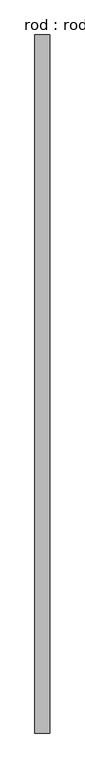
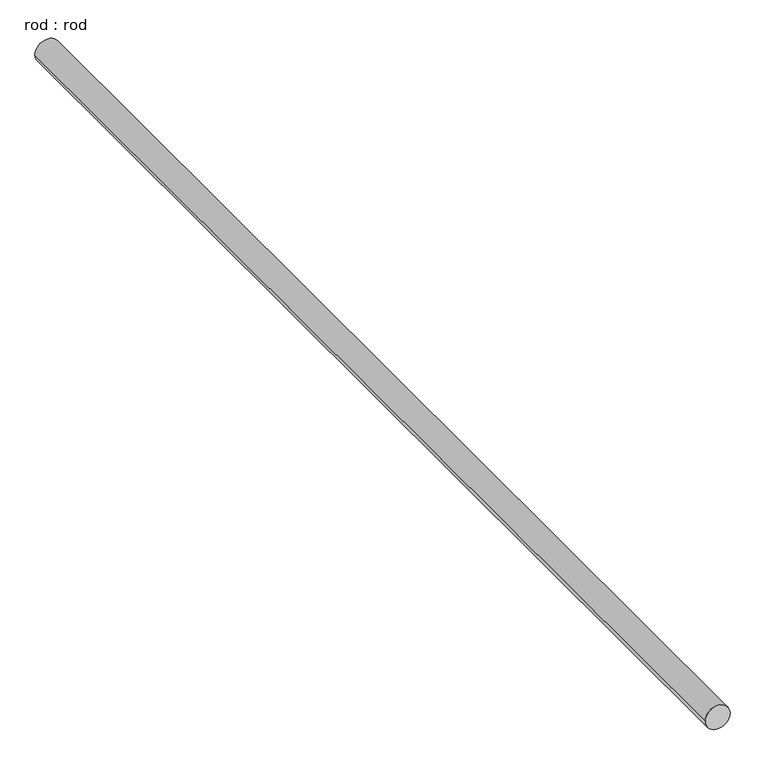
"""IFC4 building model written with IfcOpenShell, lengths in millimetres: proxy geometry, rod : rod."""

import ifcopenshell
import ifcopenshell.guid

model = None  # the IFC model being written
_history = None  # IfcOwnerHistory: only IFC2X3 demands one
_inside = {}  # id of a spatial element -> (the spatial element, [elements in it])
_under = {}  # id of a project, library or spatial element -> (it, [spatial elements below it])
_declared = {}  # id of a project -> (the project, [libraries it declares])
_typed = {}  # id of a type object -> (the type object, [elements of that type])
_made_of = {}  # id of a material, layer set ... -> (it, [elements and type objects made of it])


def new_model(schema):
    """Start an empty IFC model of exactly this schema.

    Asked for "IFC4X3", IfcOpenShell would pick the latest addendum, in which some entities
    have other attributes; the version numbers below select the first issue.
    IFC2X3 requires an IfcOwnerHistory on every rooted entity: one is made here for all.
    """
    global model, _history
    if schema == "IFC4X3":
        model = ifcopenshell.file(schema_version=(4, 3, 0, 0))
    else:
        model = ifcopenshell.file(schema=schema)
    _inside.clear()
    _under.clear()
    _declared.clear()
    _typed.clear()
    _made_of.clear()
    _history = None
    if model.schema == "IFC2X3":
        org = make("IfcOrganization", Name="unknown")
        user = make(
            "IfcPersonAndOrganization",
            ThePerson=make("IfcPerson", FamilyName="unknown"),
            TheOrganization=org,
        )
        app = make(
            "IfcApplication",
            ApplicationDeveloper=org,
            Version="unknown",
            ApplicationFullName="unknown",
            ApplicationIdentifier="unknown",
        )
        _history = make(
            "IfcOwnerHistory",
            OwningUser=user,
            OwningApplication=app,
            ChangeAction="ADDED",
            CreationDate=0,
        )
    return model


def make(cls, **values):
    """One entity of the class cls with the attributes given. An attribute that is None is left unset."""
    return model.create_entity(
        cls, **{name: value for name, value in values.items() if value is not None}
    )


def rooted(cls, **values):
    """An entity with a GlobalId (a new one), such as an element, a storey or a relation."""
    return make(cls, GlobalId=ifcopenshell.guid.new(), OwnerHistory=_history, **values)


def si_unit(unit_type, name, prefix=None):
    """IfcSIUnit, for example si_unit("LENGTHUNIT", "METRE", prefix="MILLI")."""
    return make("IfcSIUnit", UnitType=unit_type, Prefix=prefix, Name=name)


def assignment(units):
    """IfcUnitAssignment: the units of a project."""
    return None if units is None else make("IfcUnitAssignment", Units=units)


def point(xyz):
    """IfcCartesianPoint."""
    return None if xyz is None else make("IfcCartesianPoint", Coordinates=xyz)


def direction(xyz):
    """IfcDirection."""
    return None if xyz is None else make("IfcDirection", DirectionRatios=xyz)


def frame(location, z_axis=None, x_axis=None):
    """IfcAxis2Placement3D, a coordinate frame: its origin and axes. An axis left out is left unset."""
    return make(
        "IfcAxis2Placement3D",
        Location=point(location),
        Axis=direction(z_axis),
        RefDirection=direction(x_axis),
    )


def frame_2d(location, x_axis=None):
    """IfcAxis2Placement2D, a coordinate frame in the plane: its origin and x axis."""
    return make(
        "IfcAxis2Placement2D", Location=point(location), RefDirection=direction(x_axis)
    )


def origin():
    """The frame at (0, 0, 0) with its axes left unset."""
    return frame((0.0, 0.0, 0.0))


def place(relative_to, where):
    """IfcLocalPlacement: puts the frame where relative to a parent placement (None: the world)."""
    return make(
        "IfcLocalPlacement", PlacementRelTo=relative_to, RelativePlacement=where
    )


def context(
    kind, dimensions, precision=None, world=None, true_north=None, identifier=None
):
    """IfcGeometricRepresentationContext, for example the 3D "Model" context."""
    return make(
        "IfcGeometricRepresentationContext",
        ContextIdentifier=identifier,
        ContextType=kind,
        CoordinateSpaceDimension=dimensions,
        Precision=precision,
        WorldCoordinateSystem=world,
        TrueNorth=true_north,
    )


def project(units=None, contexts=None):
    """IfcProject with its units and contexts."""
    return rooted(
        "IfcProject",
        Name="project",
        RepresentationContexts=contexts,
        UnitsInContext=assignment(units),
    )


def spatial(cls, under=None, at=None, **own):
    """A site, building, storey or space (cls), placed at a placement, below another one or the project."""
    s = rooted(cls, ObjectPlacement=at, **own)
    if under is not None:
        _under.setdefault(under.id(), (under, []))[1].append(s)
    return s


def circle_curve(where, radius):
    """IfcCircle in the frame where."""
    return make("IfcCircle", Position=where, Radius=radius)


def trimmed(basis, trim1, trim2, sense, master):
    """IfcTrimmedCurve: the piece of a basis curve between two trims."""
    return make(
        "IfcTrimmedCurve",
        BasisCurve=basis,
        Trim1=trim1,
        Trim2=trim2,
        SenseAgreement=sense,
        MasterRepresentation=master,
    )


def segment(curve, same_sense, transition):
    """IfcCompositeCurveSegment."""
    return make(
        "IfcCompositeCurveSegment",
        Transition=transition,
        SameSense=same_sense,
        ParentCurve=curve,
    )


def composite_curve(segments, self_intersect=None):
    """IfcCompositeCurve: segments joined end to end."""
    return make("IfcCompositeCurve", Segments=segments, SelfIntersect=self_intersect)


def outline(outer, holes=None, kind="AREA"):
    """IfcArbitraryClosedProfileDef: a profile drawn as a closed curve; with holes, ...WithVoids."""
    if holes is None:
        return make("IfcArbitraryClosedProfileDef", ProfileType=kind, OuterCurve=outer)
    return make(
        "IfcArbitraryProfileDefWithVoids",
        ProfileType=kind,
        OuterCurve=outer,
        InnerCurves=holes,
    )


def extrude(swept, where, along, depth):
    """IfcExtrudedAreaSolid: the profile swept, set in the frame where, extruded along a direction by depth."""
    return make(
        "IfcExtrudedAreaSolid",
        SweptArea=swept,
        Position=where,
        ExtrudedDirection=direction(along),
        Depth=depth,
    )


def shape(context_of_items, identifier, shape_type, items):
    """IfcShapeRepresentation: the items that make up one representation, for example the "Body"."""
    return make(
        "IfcShapeRepresentation",
        ContextOfItems=context_of_items,
        RepresentationIdentifier=identifier,
        RepresentationType=shape_type,
        Items=items,
    )


def source(mapping_origin, context_of_items, identifier, shape_type, items):
    """IfcRepresentationMap: a shape defined once, which mapped items show again and again."""
    return make(
        "IfcRepresentationMap",
        MappingOrigin=mapping_origin,
        MappedRepresentation=shape(context_of_items, identifier, shape_type, items),
    )


def transform(
    local_origin,
    x_axis=None,
    y_axis=None,
    z_axis=None,
    scale=None,
    scale2=None,
    scale3=None,
    uniform=True,
):
    """IfcCartesianTransformationOperator3D, or its non-uniform kind. x_axis, y_axis, z_axis: its Axis1, 2, 3."""
    if uniform:
        return make(
            "IfcCartesianTransformationOperator3D",
            Axis1=direction(x_axis),
            Axis2=direction(y_axis),
            LocalOrigin=point(local_origin),
            Scale=scale,
            Axis3=direction(z_axis),
        )
    return make(
        "IfcCartesianTransformationOperator3DnonUniform",
        Axis1=direction(x_axis),
        Axis2=direction(y_axis),
        LocalOrigin=point(local_origin),
        Scale=scale,
        Axis3=direction(z_axis),
        Scale2=scale2,
        Scale3=scale3,
    )


def mapped(mapping_source, mapping_target):
    """IfcMappedItem: shows the shape of a source again, moved by a transform."""
    return make(
        "IfcMappedItem", MappingSource=mapping_source, MappingTarget=mapping_target
    )


def made_of(thing, what):
    """Note that an element or type object is made of a material, layer set ...; save() writes the relation."""
    if what is not None:
        _made_of.setdefault(what.id(), (what, []))[1].append(thing)
    return thing


def element(
    cls,
    number,
    at=None,
    inside=None,
    cuts=None,
    type_object=None,
    material=None,
    context=None,
    identifier="Body",
    shape_type=None,
    held_by="IfcProductDefinitionShape",
    body=None,
    shapes=None,
    **own,
):
    """One element of the class cls, such as IfcWall. Its Tag is "e" and its number.

    at: its placement. inside: the storey or other place that contains it. cuts: it is an
    opening in that element (IfcRelVoidsElement). A single representation is given by context,
    identifier, shape_type and body (its items); several are given by shapes. held_by: the class
    of the entity that holds the representations. save() writes the other relations.
    """
    e = rooted(cls, Tag="e%d" % number, ObjectPlacement=at, **own)
    if body is not None:
        shapes = [shape(context, identifier, shape_type, body)]
    if shapes is not None:
        e.Representation = make(held_by, Representations=shapes)
    if inside is not None:
        _inside.setdefault(inside.id(), (inside, []))[1].append(e)
    if cuts is not None:
        rooted(
            "IfcRelVoidsElement", RelatingBuildingElement=cuts, RelatedOpeningElement=e
        )
    if type_object is not None:
        _typed.setdefault(type_object.id(), (type_object, []))[1].append(e)
    return made_of(e, material)


def aggregate(whole, parts):
    """IfcRelAggregates: a whole, such as a stair, and the parts it consists of."""
    return rooted("IfcRelAggregates", RelatingObject=whole, RelatedObjects=parts)


def save(model, path):
    """Write the relations noted so far, then the file.

    IfcRelAggregates (storeys below a building ...), IfcRelContainedInSpatialStructure (elements
    in a storey), IfcRelDefinesByType, IfcRelAssociatesMaterial and IfcRelDeclares: one each for
    every whole, place, type object, material and project.
    """
    for whole, parts in _under.values():
        aggregate(whole, parts)
    for where, things in _inside.values():
        rooted(
            "IfcRelContainedInSpatialStructure",
            RelatedElements=things,
            RelatingStructure=where,
        )
    for kind, things in _typed.values():
        rooted("IfcRelDefinesByType", RelatedObjects=things, RelatingType=kind)
    for what, things in _made_of.values():
        rooted("IfcRelAssociatesMaterial", RelatedObjects=things, RelatingMaterial=what)
    for by, libraries in _declared.values():
        rooted("IfcRelDeclares", RelatingContext=by, RelatedDefinitions=libraries)
    model.write(path)


def rod_rod_a1d771e2(model_context):
    return source(origin(), model_context, "Body", "SweptSolid", [
        extrude(outline(composite_curve([segment(trimmed(circle_curve(frame_2d((0.0108462, 0.0)), 200.0), [point((0.0108462, 200.0))], [point((0.0108462, -200.0))], False, "CARTESIAN"), True, "CONTINUOUS"), segment(trimmed(circle_curve(frame_2d((0.0108462, 0.0)), 200.0), [point((0.0108462, -200.0))], [point((0.0108462, 200.0))], False, "CARTESIAN"), True, "CONTINUOUS")], self_intersect=False)), frame((0.0, -5201.9142418, 0.0), z_axis=(0.0, 1.0, 0.0), x_axis=(0.0, 0.0, 1.0)), (0.0, 0.0, 1.0), 18589.2857143),
    ])


if __name__ == "__main__":
    model = new_model("IFC4")
    model_context = context("Model", 3, world=origin())
    ifc_project = project(units=[si_unit("LENGTHUNIT", "METRE", prefix="MILLI")], contexts=[model_context])
    site = spatial("IfcSite", under=ifc_project)
    building = spatial("IfcBuilding", under=site)
    placement = place(None, origin())
    rod_rod_shape = rod_rod_a1d771e2(model_context)
    element("IfcBuildingElementProxy", 1, Name="rod : rod", ObjectType="rod : rod", at=placement, inside=building, context=model_context, shape_type="MappedRepresentation", body=[
        mapped(rod_rod_shape, transform((0.0, 0.0, 0.0), x_axis=(1.0, 0.0, 0.0), y_axis=(0.0, 1.0, 0.0), z_axis=(0.0, 0.0, 1.0))),
    ])
    save(model, "model.ifc")

# Revit data of these elements
# Type "rod : rod"
#   Default Elevation = 0
